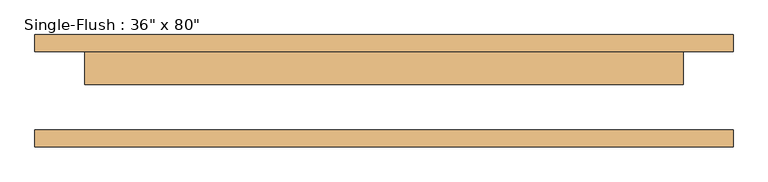
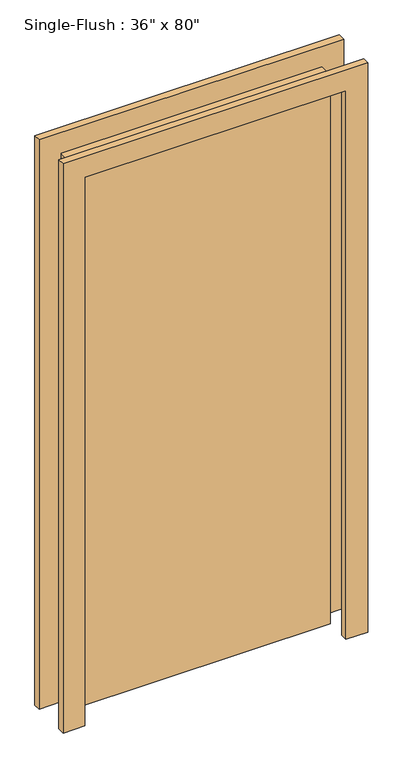
"""IFC4 building model written with IfcOpenShell, lengths in millimetres: door geometry."""

from ifc_helpers import new_model, si_unit, frame, origin, origin_with_axes, place, context, project, spatial, polyline, outline, extrude, source, transform, mapped, element, save


def door_156d4006(model_context):
    return source(origin(), model_context, "Body", "SweptSolid", [
        extrude(outline(polyline([(2108.2, -533.4), (0.0, -533.4), (0.0, -457.2), (2032.0, -457.2), (2032.0, 457.2), (0.0, 457.2), (0.0, 533.4), (2108.2, 533.4), (2108.2, -533.4)])), frame((0.0, 60.325, 0.0), z_axis=(0.0, 1.0, 0.0), x_axis=(0.0, 0.0, 1.0)), (0.0, 0.0, 1.0), 25.4),
        extrude(outline(polyline([(2108.2, 533.4), (2108.2, -533.4), (0.0, -533.4), (0.0, -457.2), (2032.0, -457.2), (2032.0, 457.2), (0.0, 457.2), (0.0, 533.4), (2108.2, 533.4)])), frame((0.0, -85.725, 0.0), z_axis=(0.0, 1.0, 0.0), x_axis=(0.0, 0.0, 1.0)), (0.0, 0.0, 1.0), 25.4),
        extrude(outline(polyline([(457.2, 9.525), (-457.2, 9.525), (-457.2, 60.325), (457.2, 60.325), (457.2, 9.525)])), origin_with_axes(), (0.0, 0.0, 1.0), 2032.0),
    ])


if __name__ == "__main__":
    model = new_model("IFC4")
    model_context = context("Model", 3, world=origin())
    ifc_project = project(units=[si_unit("LENGTHUNIT", "METRE", prefix="MILLI")], contexts=[model_context])
    site = spatial("IfcSite", under=ifc_project)
    building = spatial("IfcBuilding", under=site)
    placement = place(None, origin())
    door_shape = door_156d4006(model_context)
    element("IfcDoor", 1, ObjectType="Single-Flush : 36\" x 80\"", at=placement, inside=building, context=model_context, shape_type="MappedRepresentation", body=[
        mapped(door_shape, transform((0.0, 0.0, 0.0), x_axis=(1.0, 0.0, 0.0), y_axis=(0.0, 1.0, 0.0), z_axis=(0.0, 0.0, 1.0))),
    ])
    save(model, "model.ifc")

# Revit data of these elements
# Type "Single-Flush : 36\" x 80\""
#   Type Mark = "6"
#   Assembly Code = "C1020"
#   Thickness = 0' - 2"
#   Height = 6' - 8"
#   Trim Projection Ext = 0' - 1"
#   Trim Projection Int = 0' - 1"
#   Trim Width = 0' - 3"
#   Width = 3' - 0"
#   Door Material = drywall
#   Frame Material = drywall
#   Function = (empty or 0)
#   Wall Closure = (empty or 0)
# Element 1 (IfcDoor, "Single-Flush : 36\" x 80\"")
#   Materials on its faces: "drywall"
# Materials
#   "drywall": class "Generic", colour RGB 255 255 255, transparency 0, Description = "Gypsum Wall Board", Cost = 0
